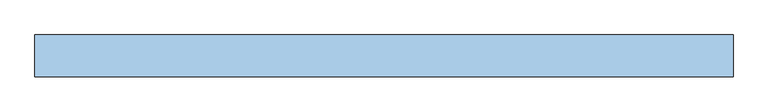
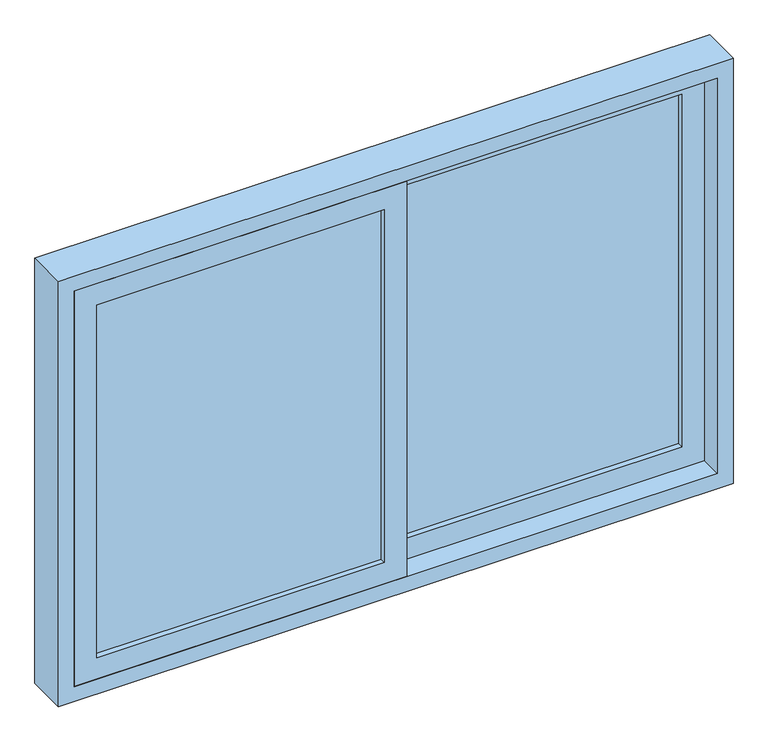
"""IFC4 building model written with IfcOpenShell, lengths in millimetres: window geometry, Janela de correr - 2 Painéis : .Janela 2 Folhas - 150x100/110."""

from ifc_helpers import new_model, si_unit, frame, origin, place, context, project, spatial, polyline, outline, extrude, source, transform, mapped, element, save


def window_fbe88107(model_context):
    return source(origin(), model_context, "Body", "SweptSolid", [
        extrude(outline(polyline([(-665.0, -73.0), (-25.0, -73.0), (-25.0, -87.0), (-665.0, -87.0), (-665.0, -73.0)])), frame((0.0, 0.0, 1185.0), z_axis=(0.0, 0.0, 1.0), x_axis=(1.0, 0.0, 0.0)), (0.0, 0.0, 1.0), 830.0),
        extrude(outline(polyline([(25.0, -23.0), (665.0, -23.0), (665.0, -37.0), (25.0, -37.0), (25.0, -23.0)])), frame((0.0, 0.0, 1185.0), z_axis=(0.0, 0.0, 1.0), x_axis=(1.0, 0.0, 0.0)), (0.0, 0.0, 1.0), 830.0),
        extrude(outline(polyline([(2100.0, 750.0), (2100.0, -750.0), (1100.0, -750.0), (1100.0, 750.0), (2100.0, 750.0)]), holes=[polyline([(1135.0, 715.0), (1135.0, -715.0), (2065.0, -715.0), (2065.0, 715.0), (1135.0, 715.0)])]), frame((0.0, -100.0, 0.0), z_axis=(0.0, 1.0, 0.0), x_axis=(0.0, 0.0, 1.0)), (0.0, 0.0, 1.0), 90.0),
        extrude(outline(polyline([(2065.0, 25.0), (2065.0, -715.0), (1135.0, -715.0), (1135.0, 25.0), (2065.0, 25.0)]), holes=[polyline([(1185.0, -25.0), (1185.0, -665.0), (2015.0, -665.0), (2015.0, -25.0), (1185.0, -25.0)])]), frame((0.0, -100.0, 0.0), z_axis=(0.0, 1.0, 0.0), x_axis=(0.0, 0.0, 1.0)), (0.0, 0.0, 1.0), 40.0),
        extrude(outline(polyline([(1135.0, -25.0), (1135.0, 715.0), (2065.0, 715.0), (2065.0, -25.0), (1135.0, -25.0)]), holes=[polyline([(2015.0, 25.0), (2015.0, 665.0), (1185.0, 665.0), (1185.0, 25.0), (2015.0, 25.0)])]), frame((0.0, -50.0, 0.0), z_axis=(0.0, 1.0, 0.0), x_axis=(0.0, 0.0, 1.0)), (0.0, 0.0, 1.0), 40.0),
    ])


if __name__ == "__main__":
    model = new_model("IFC4")
    model_context = context("Model", 3, world=origin())
    ifc_project = project(units=[si_unit("LENGTHUNIT", "METRE", prefix="MILLI")], contexts=[model_context])
    site = spatial("IfcSite", under=ifc_project)
    building = spatial("IfcBuilding", under=site)
    placement = place(None, origin())
    window_shape = window_fbe88107(model_context)
    element("IfcWindow", 1, ObjectType="Janela de correr - 2 Painéis : .Janela 2 Folhas - 150x100/110", at=placement, inside=building, context=model_context, shape_type="MappedRepresentation", body=[
        mapped(window_shape, transform((0.0, 0.0, 0.0), x_axis=(1.0, 0.0, 0.0), y_axis=(0.0, 1.0, 0.0), z_axis=(0.0, 0.0, 1.0))),
    ])
    save(model, "model.ifc")

# Revit data of these elements
# Type "Janela de correr - 2 Painéis : .Janela 2 Folhas - 150x100/110"
#   Type Mark = "20"
#   Construction Type Id = "GSP4R"
#   Analytic Construction = "Vidraça única Pilkington 1/8 pol"
#   Visual Light Transmittance = 0.9
#   Solar Heat Gain Coefficient = 0.78
#   Rough Width = 1.50 m
#   Rough Height = 1.00 m
#   Largura da moldura do painel = 0.05 m
#   Espessura da moldura do painel = 0.04 m
#   Height = 1.00 m
#   Heat Transfer Coefficient (U) = 3.6886 W/(m²·K)
#   Largura da estrutura = 0.035 m
#   Espessura da moldura = 0.09 m
#   Altura-padrão do peitoril = 1.10 m
#   Width = 1.50 m
#   Define Thermal Properties by = 1
#   Vidro = none
#   Material da moldura = none
#   Wall Closure = (empty or 0)
# Element 1 (IfcWindow, "Janela de correr - 2 Painéis : .Janela 2 Folhas - 150x100/110")
#   Materials on its faces: "Vidro"
# Materials
#   "Vidro": class "Vidro", colour RGB 0 128 192, transparency 0.9, Description = "Vidro de sílica", Cost = 0
